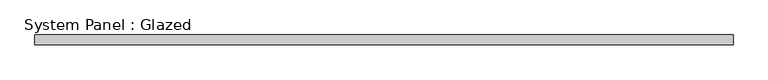
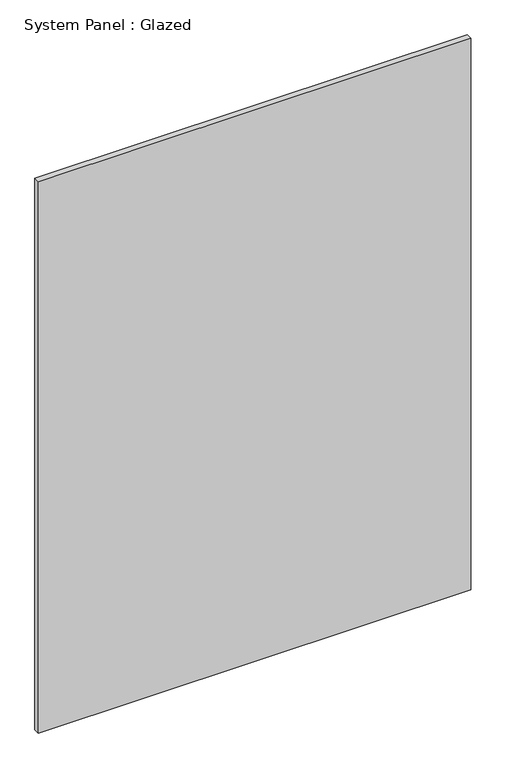
"""IFC4 building model written with IfcOpenShell, lengths in millimetres: plate geometry, System Panel : Glazed."""

import ifcopenshell
import ifcopenshell.guid

model = None  # the IFC model being written
_history = None  # IfcOwnerHistory: only IFC2X3 demands one
_inside = {}  # id of a spatial element -> (the spatial element, [elements in it])
_under = {}  # id of a project, library or spatial element -> (it, [spatial elements below it])
_declared = {}  # id of a project -> (the project, [libraries it declares])
_typed = {}  # id of a type object -> (the type object, [elements of that type])
_made_of = {}  # id of a material, layer set ... -> (it, [elements and type objects made of it])


def new_model(schema):
    """Start an empty IFC model of exactly this schema.

    Asked for "IFC4X3", IfcOpenShell would pick the latest addendum, in which some entities
    have other attributes; the version numbers below select the first issue.
    IFC2X3 requires an IfcOwnerHistory on every rooted entity: one is made here for all.
    """
    global model, _history
    if schema == "IFC4X3":
        model = ifcopenshell.file(schema_version=(4, 3, 0, 0))
    else:
        model = ifcopenshell.file(schema=schema)
    _inside.clear()
    _under.clear()
    _declared.clear()
    _typed.clear()
    _made_of.clear()
    _history = None
    if model.schema == "IFC2X3":
        org = make("IfcOrganization", Name="unknown")
        user = make(
            "IfcPersonAndOrganization",
            ThePerson=make("IfcPerson", FamilyName="unknown"),
            TheOrganization=org,
        )
        app = make(
            "IfcApplication",
            ApplicationDeveloper=org,
            Version="unknown",
            ApplicationFullName="unknown",
            ApplicationIdentifier="unknown",
        )
        _history = make(
            "IfcOwnerHistory",
            OwningUser=user,
            OwningApplication=app,
            ChangeAction="ADDED",
            CreationDate=0,
        )
    return model


def make(cls, **values):
    """One entity of the class cls with the attributes given. An attribute that is None is left unset."""
    return model.create_entity(
        cls, **{name: value for name, value in values.items() if value is not None}
    )


def rooted(cls, **values):
    """An entity with a GlobalId (a new one), such as an element, a storey or a relation."""
    return make(cls, GlobalId=ifcopenshell.guid.new(), OwnerHistory=_history, **values)


def si_unit(unit_type, name, prefix=None):
    """IfcSIUnit, for example si_unit("LENGTHUNIT", "METRE", prefix="MILLI")."""
    return make("IfcSIUnit", UnitType=unit_type, Prefix=prefix, Name=name)


def assignment(units):
    """IfcUnitAssignment: the units of a project."""
    return None if units is None else make("IfcUnitAssignment", Units=units)


def point(xyz):
    """IfcCartesianPoint."""
    return None if xyz is None else make("IfcCartesianPoint", Coordinates=xyz)


def direction(xyz):
    """IfcDirection."""
    return None if xyz is None else make("IfcDirection", DirectionRatios=xyz)


def frame(location, z_axis=None, x_axis=None):
    """IfcAxis2Placement3D, a coordinate frame: its origin and axes. An axis left out is left unset."""
    return make(
        "IfcAxis2Placement3D",
        Location=point(location),
        Axis=direction(z_axis),
        RefDirection=direction(x_axis),
    )


def origin():
    """The frame at (0, 0, 0) with its axes left unset."""
    return frame((0.0, 0.0, 0.0))


def origin_with_axes():
    """The frame at (0, 0, 0) with the z axis (0, 0, 1) and the x axis (1, 0, 0) written out."""
    return frame((0.0, 0.0, 0.0), z_axis=(0.0, 0.0, 1.0), x_axis=(1.0, 0.0, 0.0))


def place(relative_to, where):
    """IfcLocalPlacement: puts the frame where relative to a parent placement (None: the world)."""
    return make(
        "IfcLocalPlacement", PlacementRelTo=relative_to, RelativePlacement=where
    )


def context(
    kind, dimensions, precision=None, world=None, true_north=None, identifier=None
):
    """IfcGeometricRepresentationContext, for example the 3D "Model" context."""
    return make(
        "IfcGeometricRepresentationContext",
        ContextIdentifier=identifier,
        ContextType=kind,
        CoordinateSpaceDimension=dimensions,
        Precision=precision,
        WorldCoordinateSystem=world,
        TrueNorth=true_north,
    )


def project(units=None, contexts=None):
    """IfcProject with its units and contexts."""
    return rooted(
        "IfcProject",
        Name="project",
        RepresentationContexts=contexts,
        UnitsInContext=assignment(units),
    )


def spatial(cls, under=None, at=None, **own):
    """A site, building, storey or space (cls), placed at a placement, below another one or the project."""
    s = rooted(cls, ObjectPlacement=at, **own)
    if under is not None:
        _under.setdefault(under.id(), (under, []))[1].append(s)
    return s


def polyline(points):
    """IfcPolyline through the points."""
    return make("IfcPolyline", Points=[point(p) for p in points])


def outline(outer, holes=None, kind="AREA"):
    """IfcArbitraryClosedProfileDef: a profile drawn as a closed curve; with holes, ...WithVoids."""
    if holes is None:
        return make("IfcArbitraryClosedProfileDef", ProfileType=kind, OuterCurve=outer)
    return make(
        "IfcArbitraryProfileDefWithVoids",
        ProfileType=kind,
        OuterCurve=outer,
        InnerCurves=holes,
    )


def extrude(swept, where, along, depth):
    """IfcExtrudedAreaSolid: the profile swept, set in the frame where, extruded along a direction by depth."""
    return make(
        "IfcExtrudedAreaSolid",
        SweptArea=swept,
        Position=where,
        ExtrudedDirection=direction(along),
        Depth=depth,
    )


def shape(context_of_items, identifier, shape_type, items):
    """IfcShapeRepresentation: the items that make up one representation, for example the "Body"."""
    return make(
        "IfcShapeRepresentation",
        ContextOfItems=context_of_items,
        RepresentationIdentifier=identifier,
        RepresentationType=shape_type,
        Items=items,
    )


def source(mapping_origin, context_of_items, identifier, shape_type, items):
    """IfcRepresentationMap: a shape defined once, which mapped items show again and again."""
    return make(
        "IfcRepresentationMap",
        MappingOrigin=mapping_origin,
        MappedRepresentation=shape(context_of_items, identifier, shape_type, items),
    )


def transform(
    local_origin,
    x_axis=None,
    y_axis=None,
    z_axis=None,
    scale=None,
    scale2=None,
    scale3=None,
    uniform=True,
):
    """IfcCartesianTransformationOperator3D, or its non-uniform kind. x_axis, y_axis, z_axis: its Axis1, 2, 3."""
    if uniform:
        return make(
            "IfcCartesianTransformationOperator3D",
            Axis1=direction(x_axis),
            Axis2=direction(y_axis),
            LocalOrigin=point(local_origin),
            Scale=scale,
            Axis3=direction(z_axis),
        )
    return make(
        "IfcCartesianTransformationOperator3DnonUniform",
        Axis1=direction(x_axis),
        Axis2=direction(y_axis),
        LocalOrigin=point(local_origin),
        Scale=scale,
        Axis3=direction(z_axis),
        Scale2=scale2,
        Scale3=scale3,
    )


def mapped(mapping_source, mapping_target):
    """IfcMappedItem: shows the shape of a source again, moved by a transform."""
    return make(
        "IfcMappedItem", MappingSource=mapping_source, MappingTarget=mapping_target
    )


def made_of(thing, what):
    """Note that an element or type object is made of a material, layer set ...; save() writes the relation."""
    if what is not None:
        _made_of.setdefault(what.id(), (what, []))[1].append(thing)
    return thing


def element(
    cls,
    number,
    at=None,
    inside=None,
    cuts=None,
    type_object=None,
    material=None,
    context=None,
    identifier="Body",
    shape_type=None,
    held_by="IfcProductDefinitionShape",
    body=None,
    shapes=None,
    **own,
):
    """One element of the class cls, such as IfcWall. Its Tag is "e" and its number.

    at: its placement. inside: the storey or other place that contains it. cuts: it is an
    opening in that element (IfcRelVoidsElement). A single representation is given by context,
    identifier, shape_type and body (its items); several are given by shapes. held_by: the class
    of the entity that holds the representations. save() writes the other relations.
    """
    e = rooted(cls, Tag="e%d" % number, ObjectPlacement=at, **own)
    if body is not None:
        shapes = [shape(context, identifier, shape_type, body)]
    if shapes is not None:
        e.Representation = make(held_by, Representations=shapes)
    if inside is not None:
        _inside.setdefault(inside.id(), (inside, []))[1].append(e)
    if cuts is not None:
        rooted(
            "IfcRelVoidsElement", RelatingBuildingElement=cuts, RelatedOpeningElement=e
        )
    if type_object is not None:
        _typed.setdefault(type_object.id(), (type_object, []))[1].append(e)
    return made_of(e, material)


def aggregate(whole, parts):
    """IfcRelAggregates: a whole, such as a stair, and the parts it consists of."""
    return rooted("IfcRelAggregates", RelatingObject=whole, RelatedObjects=parts)


def save(model, path):
    """Write the relations noted so far, then the file.

    IfcRelAggregates (storeys below a building ...), IfcRelContainedInSpatialStructure (elements
    in a storey), IfcRelDefinesByType, IfcRelAssociatesMaterial and IfcRelDeclares: one each for
    every whole, place, type object, material and project.
    """
    for whole, parts in _under.values():
        aggregate(whole, parts)
    for where, things in _inside.values():
        rooted(
            "IfcRelContainedInSpatialStructure",
            RelatedElements=things,
            RelatingStructure=where,
        )
    for kind, things in _typed.values():
        rooted("IfcRelDefinesByType", RelatedObjects=things, RelatingType=kind)
    for what, things in _made_of.values():
        rooted("IfcRelAssociatesMaterial", RelatedObjects=things, RelatingMaterial=what)
    for by, libraries in _declared.values():
        rooted("IfcRelDeclares", RelatingContext=by, RelatedDefinitions=libraries)
    model.write(path)


def system_panel_glazed_046b630f(model_context):
    return source(origin(), model_context, "Body", "SweptSolid", [
        extrude(outline(polyline([(890.0, 24.5), (-890.0, 24.5), (-890.0, 49.5), (890.0, 49.5), (890.0, 24.5)])), origin_with_axes(), (0.0, 0.0, 1.0), 2400.0),
    ])


if __name__ == "__main__":
    model = new_model("IFC4")
    model_context = context("Model", 3, world=origin())
    ifc_project = project(units=[si_unit("LENGTHUNIT", "METRE", prefix="MILLI")], contexts=[model_context])
    site = spatial("IfcSite", under=ifc_project)
    building = spatial("IfcBuilding", under=site)
    placement = place(None, origin())
    system_panel_glazed_shape = system_panel_glazed_046b630f(model_context)
    element("IfcPlate", 1, ObjectType="System Panel : Glazed", at=placement, inside=building, context=model_context, shape_type="MappedRepresentation", body=[
        mapped(system_panel_glazed_shape, transform((0.0, 0.0, 0.0), x_axis=(1.0, 0.0, 0.0), y_axis=(0.0, 1.0, 0.0), z_axis=(0.0, 0.0, 1.0))),
    ])
    save(model, "model.ifc")

# Revit data of these elements
# Type "System Panel : Glazed"
#   Keynote = "H11"
#   Construction Type Id = "GSP4R"
#   Analytic Construction = "1/8 in Pilkington single glazing"
#   Visual Light Transmittance = 0.9
#   Solar Heat Gain Coefficient = 0.86
#   Heat Transfer Coefficient (U) = 6.7069 W/(m²·K)
#   Define Thermal Properties by = 1
# Element 1 (IfcPlate, "System Panel : Glazed")
#   Materials on its faces: "Glass"
# Materials
#   "Glass": class "Glass", colour RGB 0 128 192, transparency 0.9, Description = "Soda Lime Glass", Cost = 0
